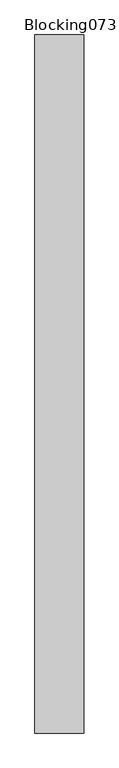
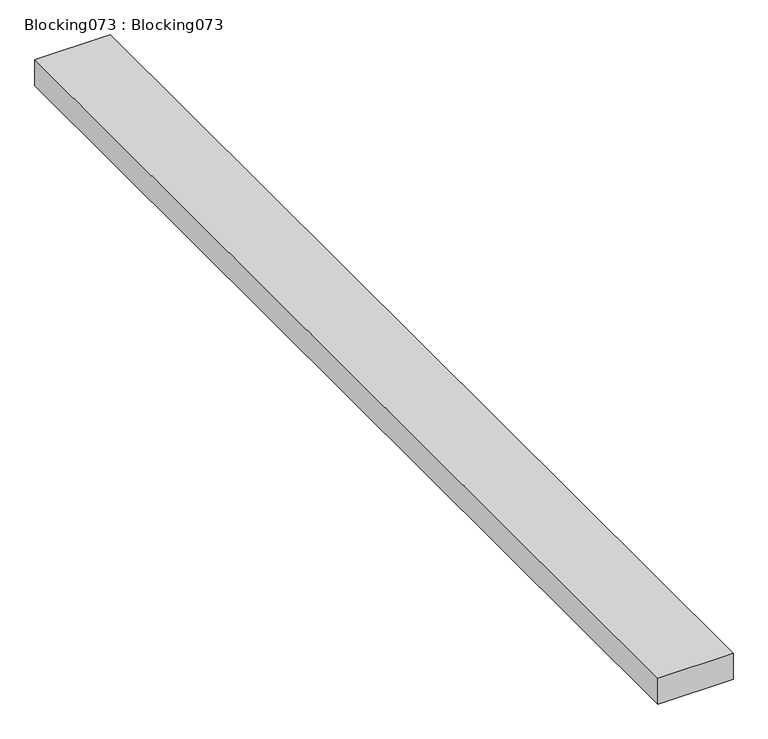
"""IFC4 building model written with IfcOpenShell, lengths in millimetres: proxy geometry, Blocking073 : Blocking073."""

import ifcopenshell
import ifcopenshell.guid

model = None  # the IFC model being written
_history = None  # IfcOwnerHistory: only IFC2X3 demands one
_inside = {}  # id of a spatial element -> (the spatial element, [elements in it])
_under = {}  # id of a project, library or spatial element -> (it, [spatial elements below it])
_declared = {}  # id of a project -> (the project, [libraries it declares])
_typed = {}  # id of a type object -> (the type object, [elements of that type])
_made_of = {}  # id of a material, layer set ... -> (it, [elements and type objects made of it])


def new_model(schema):
    """Start an empty IFC model of exactly this schema.

    Asked for "IFC4X3", IfcOpenShell would pick the latest addendum, in which some entities
    have other attributes; the version numbers below select the first issue.
    IFC2X3 requires an IfcOwnerHistory on every rooted entity: one is made here for all.
    """
    global model, _history
    if schema == "IFC4X3":
        model = ifcopenshell.file(schema_version=(4, 3, 0, 0))
    else:
        model = ifcopenshell.file(schema=schema)
    _inside.clear()
    _under.clear()
    _declared.clear()
    _typed.clear()
    _made_of.clear()
    _history = None
    if model.schema == "IFC2X3":
        org = make("IfcOrganization", Name="unknown")
        user = make(
            "IfcPersonAndOrganization",
            ThePerson=make("IfcPerson", FamilyName="unknown"),
            TheOrganization=org,
        )
        app = make(
            "IfcApplication",
            ApplicationDeveloper=org,
            Version="unknown",
            ApplicationFullName="unknown",
            ApplicationIdentifier="unknown",
        )
        _history = make(
            "IfcOwnerHistory",
            OwningUser=user,
            OwningApplication=app,
            ChangeAction="ADDED",
            CreationDate=0,
        )
    return model


def make(cls, **values):
    """One entity of the class cls with the attributes given. An attribute that is None is left unset."""
    return model.create_entity(
        cls, **{name: value for name, value in values.items() if value is not None}
    )


def rooted(cls, **values):
    """An entity with a GlobalId (a new one), such as an element, a storey or a relation."""
    return make(cls, GlobalId=ifcopenshell.guid.new(), OwnerHistory=_history, **values)


def si_unit(unit_type, name, prefix=None):
    """IfcSIUnit, for example si_unit("LENGTHUNIT", "METRE", prefix="MILLI")."""
    return make("IfcSIUnit", UnitType=unit_type, Prefix=prefix, Name=name)


def assignment(units):
    """IfcUnitAssignment: the units of a project."""
    return None if units is None else make("IfcUnitAssignment", Units=units)


def point(xyz):
    """IfcCartesianPoint."""
    return None if xyz is None else make("IfcCartesianPoint", Coordinates=xyz)


def direction(xyz):
    """IfcDirection."""
    return None if xyz is None else make("IfcDirection", DirectionRatios=xyz)


def frame(location, z_axis=None, x_axis=None):
    """IfcAxis2Placement3D, a coordinate frame: its origin and axes. An axis left out is left unset."""
    return make(
        "IfcAxis2Placement3D",
        Location=point(location),
        Axis=direction(z_axis),
        RefDirection=direction(x_axis),
    )


def origin():
    """The frame at (0, 0, 0) with its axes left unset."""
    return frame((0.0, 0.0, 0.0))


def place(relative_to, where):
    """IfcLocalPlacement: puts the frame where relative to a parent placement (None: the world)."""
    return make(
        "IfcLocalPlacement", PlacementRelTo=relative_to, RelativePlacement=where
    )


def context(
    kind, dimensions, precision=None, world=None, true_north=None, identifier=None
):
    """IfcGeometricRepresentationContext, for example the 3D "Model" context."""
    return make(
        "IfcGeometricRepresentationContext",
        ContextIdentifier=identifier,
        ContextType=kind,
        CoordinateSpaceDimension=dimensions,
        Precision=precision,
        WorldCoordinateSystem=world,
        TrueNorth=true_north,
    )


def project(units=None, contexts=None):
    """IfcProject with its units and contexts."""
    return rooted(
        "IfcProject",
        Name="project",
        RepresentationContexts=contexts,
        UnitsInContext=assignment(units),
    )


def spatial(cls, under=None, at=None, **own):
    """A site, building, storey or space (cls), placed at a placement, below another one or the project."""
    s = rooted(cls, ObjectPlacement=at, **own)
    if under is not None:
        _under.setdefault(under.id(), (under, []))[1].append(s)
    return s


def polyline(points):
    """IfcPolyline through the points."""
    return make("IfcPolyline", Points=[point(p) for p in points])


def outline(outer, holes=None, kind="AREA"):
    """IfcArbitraryClosedProfileDef: a profile drawn as a closed curve; with holes, ...WithVoids."""
    if holes is None:
        return make("IfcArbitraryClosedProfileDef", ProfileType=kind, OuterCurve=outer)
    return make(
        "IfcArbitraryProfileDefWithVoids",
        ProfileType=kind,
        OuterCurve=outer,
        InnerCurves=holes,
    )


def extrude(swept, where, along, depth):
    """IfcExtrudedAreaSolid: the profile swept, set in the frame where, extruded along a direction by depth."""
    return make(
        "IfcExtrudedAreaSolid",
        SweptArea=swept,
        Position=where,
        ExtrudedDirection=direction(along),
        Depth=depth,
    )


def shape(context_of_items, identifier, shape_type, items):
    """IfcShapeRepresentation: the items that make up one representation, for example the "Body"."""
    return make(
        "IfcShapeRepresentation",
        ContextOfItems=context_of_items,
        RepresentationIdentifier=identifier,
        RepresentationType=shape_type,
        Items=items,
    )


def source(mapping_origin, context_of_items, identifier, shape_type, items):
    """IfcRepresentationMap: a shape defined once, which mapped items show again and again."""
    return make(
        "IfcRepresentationMap",
        MappingOrigin=mapping_origin,
        MappedRepresentation=shape(context_of_items, identifier, shape_type, items),
    )


def transform(
    local_origin,
    x_axis=None,
    y_axis=None,
    z_axis=None,
    scale=None,
    scale2=None,
    scale3=None,
    uniform=True,
):
    """IfcCartesianTransformationOperator3D, or its non-uniform kind. x_axis, y_axis, z_axis: its Axis1, 2, 3."""
    if uniform:
        return make(
            "IfcCartesianTransformationOperator3D",
            Axis1=direction(x_axis),
            Axis2=direction(y_axis),
            LocalOrigin=point(local_origin),
            Scale=scale,
            Axis3=direction(z_axis),
        )
    return make(
        "IfcCartesianTransformationOperator3DnonUniform",
        Axis1=direction(x_axis),
        Axis2=direction(y_axis),
        LocalOrigin=point(local_origin),
        Scale=scale,
        Axis3=direction(z_axis),
        Scale2=scale2,
        Scale3=scale3,
    )


def mapped(mapping_source, mapping_target):
    """IfcMappedItem: shows the shape of a source again, moved by a transform."""
    return make(
        "IfcMappedItem", MappingSource=mapping_source, MappingTarget=mapping_target
    )


def made_of(thing, what):
    """Note that an element or type object is made of a material, layer set ...; save() writes the relation."""
    if what is not None:
        _made_of.setdefault(what.id(), (what, []))[1].append(thing)
    return thing


def element(
    cls,
    number,
    at=None,
    inside=None,
    cuts=None,
    type_object=None,
    material=None,
    context=None,
    identifier="Body",
    shape_type=None,
    held_by="IfcProductDefinitionShape",
    body=None,
    shapes=None,
    **own,
):
    """One element of the class cls, such as IfcWall. Its Tag is "e" and its number.

    at: its placement. inside: the storey or other place that contains it. cuts: it is an
    opening in that element (IfcRelVoidsElement). A single representation is given by context,
    identifier, shape_type and body (its items); several are given by shapes. held_by: the class
    of the entity that holds the representations. save() writes the other relations.
    """
    e = rooted(cls, Tag="e%d" % number, ObjectPlacement=at, **own)
    if body is not None:
        shapes = [shape(context, identifier, shape_type, body)]
    if shapes is not None:
        e.Representation = make(held_by, Representations=shapes)
    if inside is not None:
        _inside.setdefault(inside.id(), (inside, []))[1].append(e)
    if cuts is not None:
        rooted(
            "IfcRelVoidsElement", RelatingBuildingElement=cuts, RelatedOpeningElement=e
        )
    if type_object is not None:
        _typed.setdefault(type_object.id(), (type_object, []))[1].append(e)
    return made_of(e, material)


def aggregate(whole, parts):
    """IfcRelAggregates: a whole, such as a stair, and the parts it consists of."""
    return rooted("IfcRelAggregates", RelatingObject=whole, RelatedObjects=parts)


def save(model, path):
    """Write the relations noted so far, then the file.

    IfcRelAggregates (storeys below a building ...), IfcRelContainedInSpatialStructure (elements
    in a storey), IfcRelDefinesByType, IfcRelAssociatesMaterial and IfcRelDeclares: one each for
    every whole, place, type object, material and project.
    """
    for whole, parts in _under.values():
        aggregate(whole, parts)
    for where, things in _inside.values():
        rooted(
            "IfcRelContainedInSpatialStructure",
            RelatedElements=things,
            RelatingStructure=where,
        )
    for kind, things in _typed.values():
        rooted("IfcRelDefinesByType", RelatedObjects=things, RelatingType=kind)
    for what, things in _made_of.values():
        rooted("IfcRelAssociatesMaterial", RelatedObjects=things, RelatingMaterial=what)
    for by, libraries in _declared.values():
        rooted("IfcRelDeclares", RelatingContext=by, RelatedDefinitions=libraries)
    model.write(path)


def blocking073_blocking073_0a36fdc9(model_context):
    return source(origin(), model_context, "Body", "SweptSolid", [
        extrude(outline(polyline([(-950.3815411, -1052.8908936), (-1090.0815411, -1052.8908936), (-1090.0815411, 947.1091064), (-950.3815411, 947.1091064), (-950.3815411, -1052.8908936)])), frame((0.0, 0.0, 40214.296), z_axis=(0.0, 0.0, 1.0), x_axis=(1.0, 0.0, 0.0)), (0.0, 0.0, 1.0), 50.8),
    ])


if __name__ == "__main__":
    model = new_model("IFC4")
    model_context = context("Model", 3, world=origin())
    ifc_project = project(units=[si_unit("LENGTHUNIT", "METRE", prefix="MILLI")], contexts=[model_context])
    site = spatial("IfcSite", under=ifc_project)
    building = spatial("IfcBuilding", under=site)
    placement = place(None, origin())
    blocking073_blocking073_shape = blocking073_blocking073_0a36fdc9(model_context)
    element("IfcBuildingElementProxy", 1, Name="Blocking073 : Blocking073", ObjectType="Blocking073 : Blocking073", at=placement, inside=building, context=model_context, shape_type="MappedRepresentation", body=[
        mapped(blocking073_blocking073_shape, transform((0.0, 0.0, 0.0), x_axis=(1.0, 0.0, 0.0), y_axis=(0.0, 1.0, 0.0), z_axis=(0.0, 0.0, 1.0))),
    ])
    save(model, "model.ifc")

# Revit data of these elements
# Type "Blocking073 : Blocking073"
#   NameOverride = "Blocking073"
# Element 1 (IfcBuildingElementProxy, "Blocking073 : Blocking073")
#   Materials on its faces: "WOOD BLOCKING AS REQUIRED"
# Materials
#   "WOOD BLOCKING AS REQUIRED": class "Unassigned", colour RGB 166 124 85, transparency 0, Cost = 0
